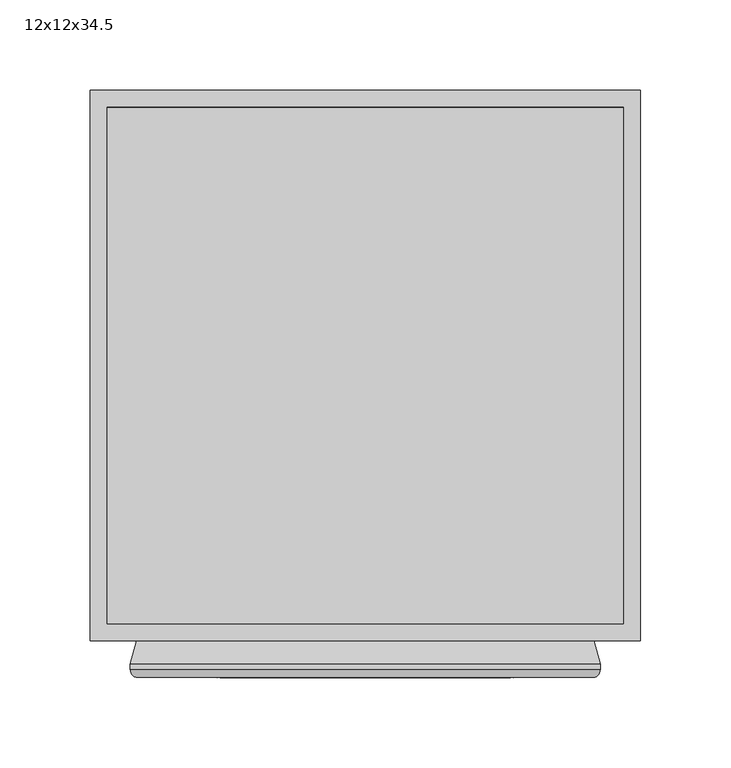
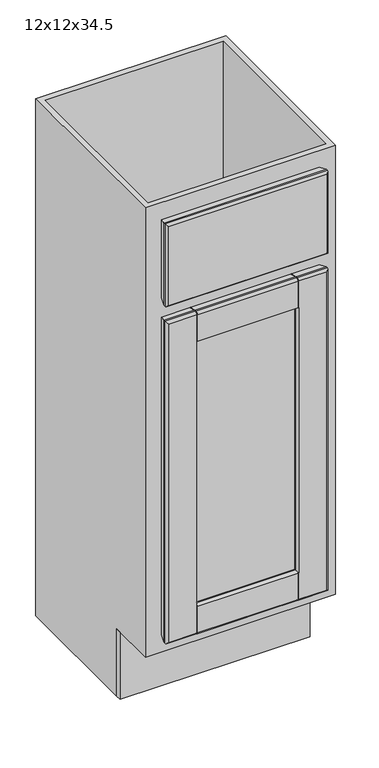
"""IFC4 building model written with IfcOpenShell, lengths in millimetres: furniture geometry, Cabinet-Base-Merillat-Single_Door-Marlin : 12x12x34.5."""

from ifc_helpers import new_model, si_unit, frame, origin, origin_with_axes, place, context, project, spatial, polyline, circle_curve, ellipse_curve, outline, extrude, faceted_brep, source, transform, mapped, element, save
from ifc_brep_helpers import plane_surface, cylinder_surface, advanced_brep


def furniture_12x12x34_5_5e3fd0ca(model_context):
    return source(origin(), model_context, "Body", "SolidModel", [
        advanced_brep(
        [(148.9127049, -625.4496, 685.8), (145.8162124, -629.92, 682.7035075), (145.8162124, -629.92, 142.7964925), (148.9127049, -625.4496, 139.7), (148.9127049, -622.681, 139.7), (148.9127049, -622.681, 685.8), (145.4075049, -609.6, 143.2052), (145.4075049, -609.6, 682.2948), (100.7115422, -609.6, 637.5988372), (100.7115422, -609.6, 187.9011628), (100.3414105, -610.39375, 188.2712945), (98.2602514, -614.85681, 190.3524535), (98.2602514, -614.85681, 635.1475465), (100.3414105, -610.39375, 637.2287055), (99.6600209, -617.0969093, 188.952684), (99.6600209, -617.0969093, 636.547316), (113.9877049, -617.347, 174.625), (113.9877049, -617.347, 650.875), (113.9877049, -622.173, 174.625), (113.9877049, -622.173, 650.875), (99.6600209, -622.4230907, 188.952684), (99.6600209, -622.4230907, 636.547316), (98.2602514, -624.66319, 190.3524535), (98.2602514, -624.66319, 635.1475465), (100.3414105, -629.12625, 188.2712945), (100.7086747, -629.9138508, 187.9040302), (100.7115422, -629.92, 637.5988372), (100.3414105, -629.12625, 637.2287055), (100.7086747, -629.92, 142.7964925), (100.7086747, -625.4496, 139.7), (-108.3408026, -629.92, 142.7964925), (-111.4372951, -625.4496, 139.7), (-63.2730764, -625.4496, 139.7), (-63.2730764, -629.92, 142.7964925), (99.1211747, -625.4496, 139.7), (99.1211747, -629.92, 142.7964925), (-61.6855764, -629.92, 142.7964925), (-61.6855764, -625.4496, 139.7), (100.7086747, -622.681, 139.7), (-111.4372951, -622.681, 139.7), (-63.2730764, -622.681, 139.7), (99.1211747, -622.681, 139.7), (-61.6855764, -622.681, 139.7), (100.7086747, -609.6, 143.2052), (-107.9320951, -609.6, 143.2052), (-63.2730764, -609.6, 143.2052), (99.1211747, -609.6, 143.2052), (-61.6855764, -609.6, 143.2052), (-60.7848416, -614.85681, 190.3524535), (99.1211747, -610.39375, 188.2712945), (99.1211747, -609.6, 187.9011628), (-61.6855764, -609.6, 187.9011628), (-61.6855764, -610.39375, 188.2712945), (-62.8660006, -610.39375, 188.2712945), (-62.184611, -617.0969093, 188.952684), (-76.5122951, -617.347, 174.625), (-76.5122951, -622.173, 174.625), (-62.184611, -622.4230907, 188.952684), (-60.7848416, -624.66319, 190.3524535), (-62.8660006, -629.12625, 188.2712945), (-61.6855764, -629.12625, 188.2712945), (-61.6855764, -629.92, 187.9011628), (99.1211747, -629.92, 187.9011628), (99.1211747, -629.12625, 188.2712945), (-108.3408026, -629.92, 682.7035075), (-111.4372951, -625.4496, 685.8), (-111.4372951, -622.681, 685.8), (-107.9320951, -609.6, 682.2948), (-63.2361323, -609.6, 187.9011628), (-63.2361323, -609.6, 637.5988372), (-62.8660006, -610.39375, 637.2287055), (-60.7848416, -614.85681, 635.1475465), (-62.184611, -617.0969093, 636.547316), (-76.5122951, -617.347, 650.875), (-76.5122951, -622.173, 650.875), (-62.184611, -622.4230907, 636.547316), (-60.7848416, -624.66319, 635.1475465), (-62.8660006, -629.12625, 637.2287055), (-63.2361323, -629.92, 637.5988372), (-63.2361323, -629.92, 187.9011628), (-63.2730764, -629.92, 682.7035075), (-63.2730764, -625.4496, 685.8), (100.7086747, -625.4496, 685.8), (100.7086747, -629.92, 682.7035075), (-61.6855764, -625.4496, 685.8), (-61.6855764, -629.92, 682.7035075), (99.1211747, -629.92, 682.7035075), (99.1211747, -625.4496, 685.8), (-63.2730764, -622.681, 685.8), (100.7086747, -622.681, 685.8), (-61.6855764, -622.681, 685.8), (99.1211747, -622.681, 685.8), (-63.2730764, -609.6, 682.2948), (100.7086747, -609.6, 682.2948), (-61.6855764, -609.6, 682.2948), (99.1211747, -609.6, 682.2948), (-61.6855764, -609.6, 637.5988372), (99.1211747, -609.6, 637.5988372), (-61.6855764, -610.39375, 637.2287055), (99.1211747, -610.39375, 637.2287055), (99.1211747, -629.12625, 637.2287055), (99.1211747, -629.92, 637.5988372), (-61.6855764, -629.92, 637.5988372), (-61.6855764, -629.12625, 637.2287055), (-61.6855764, -610.39375, 681.6857412), (-61.6855764, -622.7855037, 685.00625), (-61.6855764, -625.4496, 685.00625), (-61.6855764, -629.12625, 682.5526052), (-63.2730764, -629.12625, 637.2287055), (-63.2730764, -629.12625, 682.5526052), (-63.2730764, -625.4496, 685.00625), (-63.2730764, -622.7855037, 685.00625), (-63.2730764, -610.39375, 681.6857412), (-63.2730764, -610.39375, 637.2287055), (100.7086747, -610.39375, 637.2287055), (100.7086747, -610.39375, 681.6857412), (100.7086747, -622.7855037, 685.00625), (100.7086747, -625.4496, 685.00625), (100.7086747, -629.12625, 682.5526052), (100.7086747, -629.12625, 637.2287055), (99.1211747, -629.12625, 682.5526052), (99.1211747, -625.4496, 685.00625), (99.1211747, -622.7855037, 685.00625), (99.1211747, -610.39375, 681.6857412), (100.7086747, -629.12625, 188.2712945), (100.7086747, -629.12625, 142.9473948), (100.7086747, -625.4496, 140.49375), (100.7086747, -622.7855037, 140.49375), (100.7086747, -610.39375, 143.8142588), (100.7086747, -610.39375, 188.2712945), (99.1211747, -610.39375, 143.8142588), (99.1211747, -622.7855037, 140.49375), (99.1211747, -625.4496, 140.49375), (99.1211747, -629.12625, 142.9473948), (-61.6855764, -629.12625, 142.9473948), (-61.6855764, -625.4496, 140.49375), (-61.6855764, -622.7855037, 140.49375), (-61.6855764, -610.39375, 143.8142588), (-63.2730764, -629.12625, 188.2712945), (-63.2730764, -610.39375, 188.2712945), (-63.2730764, -610.39375, 143.8142588), (-63.2730764, -622.7855037, 140.49375), (-63.2730764, -625.4496, 140.49375), (-63.2730764, -629.12625, 142.9473948)],
        [
            (0, 1, ellipse_curve(frame((144.1375049, -625.4496, 681.0248), z_axis=(0.7071067811865475, 0.0, -0.7071067811865475), x_axis=(0.7071067811865474, 0.0, 0.7071067811865476)), 6.7531526, 4.7752)),
            (1, 2),
            (2, 3, ellipse_curve(frame((144.1375049, -625.4496, 144.4752), z_axis=(0.7071067811865475, 0.0, 0.7071067811865475), x_axis=(-0.7071067811865474, 0.0, 0.7071067811865476)), 6.7531526, 4.7752)),
            (3, 0),
            (3, 4),
            (4, 5),
            (5, 0),
            (4, 6),
            (6, 7),
            (7, 5),
            (8, 9),
            (9, 10),
            (10, 11),
            (11, 12),
            (12, 13),
            (13, 8),
            (11, 14, ellipse_curve(frame((99.6875049, -615.5223492, 188.9252), z_axis=(0.7071067811865475, 0.0, 0.7071067811865475), x_axis=(-0.7071067811865474, 0.0, 0.7071067811865476)), 2.2271035, 1.5748)),
            (14, 15),
            (15, 12, ellipse_curve(frame((99.6875049, -615.5223492, 636.5748), z_axis=(0.7071067811865475, 0.0, -0.7071067811865475), x_axis=(0.7071067811865474, 0.0, 0.7071067811865476)), 2.2271035, 1.5748)),
            (14, 16),
            (16, 17),
            (17, 15),
            (16, 18),
            (18, 19),
            (19, 17),
            (18, 20),
            (20, 21),
            (21, 19),
            (20, 22, ellipse_curve(frame((99.6875049, -623.9976508, 188.9252), z_axis=(0.7071067811865475, 0.0, 0.7071067811865475), x_axis=(-0.7071067811865474, 0.0, 0.7071067811865476)), 2.2271035, 1.5748)),
            (22, 23),
            (23, 21, ellipse_curve(frame((99.6875049, -623.9976508, 636.5748), z_axis=(0.7071067811865475, 0.0, -0.7071067811865475), x_axis=(0.7071067811865474, 0.0, 0.7071067811865476)), 2.2271035, 1.5748)),
            (22, 24),
            (24, 25),
            (25, 26),
            (26, 27),
            (27, 23),
            (2, 28),
            (28, 29, circle_curve(frame((100.7086747, -625.4496, 144.4752), z_axis=(1.0, 0.0, 0.0), x_axis=(0.0, 1.0, 0.0)), 4.7752)),
            (29, 3),
            (30, 31, ellipse_curve(frame((-106.6620951, -625.4496, 144.4752), z_axis=(0.7071067811865475, 0.0, -0.7071067811865475), x_axis=(0.7071067811865476, 0.0, 0.7071067811865474)), 6.7531526, 4.7752)),
            (31, 32),
            (32, 33, circle_curve(frame((-63.2730764, -625.4496, 144.4752), z_axis=(-1.0, 0.0, 0.0), x_axis=(0.0, 1.0, 0.0)), 4.7752)),
            (33, 30),
            (34, 35, circle_curve(frame((99.1211747, -625.4496, 144.4752), z_axis=(-1.0, 0.0, 0.0), x_axis=(0.0, 1.0, 0.0)), 4.7752)),
            (35, 36),
            (36, 37, circle_curve(frame((-61.6855764, -625.4496, 144.4752), z_axis=(1.0, 0.0, 0.0), x_axis=(0.0, 1.0, 0.0)), 4.7752)),
            (37, 34),
            (29, 38),
            (38, 4),
            (31, 39),
            (39, 40),
            (40, 32),
            (41, 34),
            (37, 42),
            (42, 41),
            (38, 43),
            (43, 6),
            (39, 44),
            (44, 45),
            (45, 40),
            (46, 41),
            (42, 47),
            (47, 46),
            (48, 11),
            (10, 49),
            (49, 50),
            (50, 51),
            (51, 52),
            (52, 53),
            (53, 48),
            (48, 54, ellipse_curve(frame((-62.2120951, -615.5223492, 188.9252), z_axis=(0.7071067811865475, 0.0, -0.7071067811865475), x_axis=(0.7071067811865476, 0.0, 0.7071067811865474)), 2.2271035, 1.5748)),
            (54, 14),
            (54, 55),
            (55, 16),
            (55, 56),
            (56, 18),
            (56, 57),
            (57, 20),
            (57, 58, ellipse_curve(frame((-62.2120951, -623.9976508, 188.9252), z_axis=(0.7071067811865475, 0.0, -0.7071067811865475), x_axis=(0.7071067811865476, 0.0, 0.7071067811865474)), 2.2271035, 1.5748)),
            (58, 22),
            (58, 59),
            (59, 60),
            (60, 61),
            (61, 62),
            (62, 63),
            (63, 24),
            (30, 64),
            (64, 65, ellipse_curve(frame((-106.6620951, -625.4496, 681.0248), z_axis=(-0.7071067811865475, 0.0, -0.7071067811865475), x_axis=(0.7071067811865474, 0.0, -0.7071067811865476)), 6.7531526, 4.7752)),
            (65, 31),
            (65, 66),
            (66, 39),
            (66, 67),
            (67, 44),
            (68, 69),
            (69, 70),
            (70, 71),
            (71, 48),
            (53, 68),
            (71, 72, ellipse_curve(frame((-62.2120951, -615.5223492, 636.5748), z_axis=(-0.7071067811865475, 0.0, -0.7071067811865475), x_axis=(0.7071067811865474, 0.0, -0.7071067811865476)), 2.2271035, 1.5748)),
            (72, 54),
            (72, 73),
            (73, 55),
            (73, 74),
            (74, 56),
            (74, 75),
            (75, 57),
            (75, 76, ellipse_curve(frame((-62.2120951, -623.9976508, 636.5748), z_axis=(-0.7071067811865475, 0.0, -0.7071067811865475), x_axis=(0.7071067811865474, 0.0, -0.7071067811865476)), 2.2271035, 1.5748)),
            (76, 58),
            (76, 77),
            (77, 78),
            (78, 79),
            (79, 59),
            (64, 80),
            (80, 81, circle_curve(frame((-63.2730764, -625.4496, 681.0248), z_axis=(-1.0, 0.0, 0.0), x_axis=(0.0, 1.0, 0.0)), 4.7752)),
            (81, 65),
            (0, 82),
            (82, 83, circle_curve(frame((100.7086747, -625.4496, 681.0248), z_axis=(1.0, 0.0, 0.0), x_axis=(0.0, 1.0, 0.0)), 4.7752)),
            (83, 1),
            (84, 85, circle_curve(frame((-61.6855764, -625.4496, 681.0248), z_axis=(1.0, 0.0, 0.0), x_axis=(0.0, 1.0, 0.0)), 4.7752)),
            (85, 86),
            (86, 87, circle_curve(frame((99.1211747, -625.4496, 681.0248), z_axis=(-1.0, 0.0, 0.0), x_axis=(0.0, 1.0, 0.0)), 4.7752)),
            (87, 84),
            (81, 88),
            (88, 66),
            (5, 89),
            (89, 82),
            (90, 84),
            (87, 91),
            (91, 90),
            (88, 92),
            (92, 67),
            (7, 93),
            (93, 89),
            (94, 90),
            (91, 95),
            (95, 94),
            (43, 9),
            (8, 93),
            (92, 69),
            (68, 45),
            (96, 94),
            (95, 97),
            (97, 96),
            (50, 46),
            (47, 51),
            (12, 71),
            (70, 98),
            (98, 96),
            (97, 99),
            (99, 13),
            (15, 72),
            (17, 73),
            (19, 74),
            (21, 75),
            (23, 76),
            (27, 100),
            (100, 101),
            (101, 102),
            (102, 103),
            (103, 77),
            (83, 26),
            (25, 28),
            (33, 79),
            (78, 80),
            (85, 102),
            (101, 86),
            (35, 62),
            (61, 36),
            (98, 104),
            (104, 105),
            (105, 106),
            (106, 107, circle_curve(frame((-61.6855764, -625.4496, 681.0248), z_axis=(1.0, 0.0, 0.0), x_axis=(0.0, 0.0, 1.0)), 3.98145)),
            (107, 103),
            (78, 108),
            (108, 109),
            (109, 110, circle_curve(frame((-63.2730764, -625.4496, 681.0248), z_axis=(-1.0, 0.0, 0.0), x_axis=(0.0, 0.0, 1.0)), 3.98145)),
            (110, 111),
            (111, 112),
            (112, 113),
            (113, 69),
            (77, 108),
            (107, 109),
            (106, 110),
            (105, 111),
            (104, 112),
            (70, 113),
            (8, 114),
            (114, 115),
            (115, 116),
            (116, 117),
            (117, 118, circle_curve(frame((100.7086747, -625.4496, 681.0248), z_axis=(1.0, 0.0, 0.0), x_axis=(0.0, 0.0, 1.0)), 3.98145)),
            (118, 119),
            (119, 26),
            (100, 120),
            (120, 121, circle_curve(frame((99.1211747, -625.4496, 681.0248), z_axis=(-1.0, 0.0, 0.0), x_axis=(0.0, 0.0, 1.0)), 3.98145)),
            (121, 122),
            (122, 123),
            (123, 99),
            (119, 27),
            (118, 120),
            (117, 121),
            (116, 122),
            (115, 123),
            (114, 13),
            (25, 124),
            (124, 125),
            (125, 126, circle_curve(frame((100.7086747, -625.4496, 144.4752), z_axis=(1.0, 0.0, 0.0), x_axis=(0.0, 0.0, 1.0)), 3.98145)),
            (126, 127),
            (127, 128),
            (128, 129),
            (129, 9),
            (49, 130),
            (130, 131),
            (131, 132),
            (132, 133, circle_curve(frame((99.1211747, -625.4496, 144.4752), z_axis=(-1.0, 0.0, 0.0), x_axis=(0.0, 0.0, 1.0)), 3.98145)),
            (133, 63),
            (129, 10),
            (128, 130),
            (127, 131),
            (126, 132),
            (125, 133),
            (124, 24),
            (60, 134),
            (134, 135, circle_curve(frame((-61.6855764, -625.4496, 144.4752), z_axis=(1.0, 0.0, 0.0), x_axis=(0.0, 0.0, 1.0)), 3.98145)),
            (135, 136),
            (136, 137),
            (137, 52),
            (138, 79),
            (68, 139),
            (139, 140),
            (140, 141),
            (141, 142),
            (142, 143, circle_curve(frame((-63.2730764, -625.4496, 144.4752), z_axis=(-1.0, 0.0, 0.0), x_axis=(0.0, 0.0, 1.0)), 3.98145)),
            (143, 138),
            (138, 59),
            (53, 139),
            (137, 140),
            (136, 141),
            (135, 142),
            (134, 143),
        ],
        [
            cylinder_surface(frame((144.1375049, -625.4496, 685.8), z_axis=(0.0, 0.0, 1.0), x_axis=(0.0, 1.0, 0.0)), 4.7752),
            plane_surface(frame((148.9127049, -625.4496, 685.8), z_axis=(1.0, 0.0, 0.0), x_axis=(0.0, 0.0, -1.0))),
            plane_surface(frame((148.9127049, -622.681, 685.8), z_axis=(0.9659229350723619, 0.25882983502910506, 0.0), x_axis=(0.0, 0.0, -1.0))),
            plane_surface(frame((100.7115422, -609.6, 637.5988372), z_axis=(-0.9063077870366099, 0.4226182617407856, 0.0), x_axis=(0.0, 0.0, -1.0))),
            cylinder_surface(frame((99.6875049, -615.5223492, 685.8), z_axis=(0.0, 0.0, 1.0000000000000002), x_axis=(-0.01745240643729364, -0.9998476951563912, 0.0)), 1.5748),
            plane_surface(frame((99.6600209, -617.0969093, 636.547316), z_axis=(-0.017452406437322144, -0.9998476951563906, 0.0), x_axis=(0.0, 0.0, -1.0))),
            plane_surface(frame((113.9877049, -617.347, 650.875), z_axis=(-1.0, 0.0, 0.0), x_axis=(0.0, 0.0, -1.0))),
            plane_surface(frame((113.9877049, -622.173, 650.875), z_axis=(-0.01745240643727848, 0.9998476951563914, 0.0), x_axis=(0.0, 0.0, -1.0))),
            cylinder_surface(frame((99.6875049, -623.9976508, 685.8), z_axis=(0.0, 0.0, 1.0000000000000002), x_axis=(-0.9063077870367326, -0.42261826174052236, 0.0)), 1.5748),
            plane_surface(frame((98.2602514, -624.66319, 635.1475465), z_axis=(-0.9063077870366333, -0.4226182617407352, 0.0), x_axis=(0.0, 0.0, -1.0))),
            cylinder_surface(frame((148.9127049, -625.4496, 144.4752), z_axis=(1.0, 0.0, 0.0), x_axis=(0.0, 1.0, 0.0)), 4.7752),
            plane_surface(frame((148.9127049, -625.4496, 139.7), z_axis=(0.0, 0.0, -1.0), x_axis=(-1.0, 0.0, 0.0))),
            plane_surface(frame((148.9127049, -622.681, 139.7), z_axis=(0.0, 0.25882983502910506, -0.9659229350723619), x_axis=(-1.0, 0.0, 0.0))),
            plane_surface(frame((100.7115422, -609.6, 187.9011628), z_axis=(0.0, 0.4226182617407856, 0.9063077870366099), x_axis=(-1.0, 0.0, 0.0))),
            cylinder_surface(frame((148.9127049, -615.5223492, 188.9252), z_axis=(1.0000000000000002, 0.0, 0.0), x_axis=(0.0, -0.9998476951563912, 0.01745240643729364)), 1.5748),
            plane_surface(frame((99.6600209, -617.0969093, 188.952684), z_axis=(0.0, -0.9998476951563906, 0.017452406437322144), x_axis=(-1.0, 0.0, 0.0))),
            plane_surface(frame((113.9877049, -617.347, 174.625), z_axis=(0.0, 0.0, 1.0), x_axis=(-1.0, 0.0, 0.0))),
            plane_surface(frame((113.9877049, -622.173, 174.625), z_axis=(0.0, 0.9998476951563914, 0.01745240643727848), x_axis=(-1.0, 0.0, 0.0))),
            cylinder_surface(frame((148.9127049, -623.9976508, 188.9252), z_axis=(1.0000000000000002, 0.0, 0.0), x_axis=(0.0, -0.42261826174052236, 0.9063077870367326)), 1.5748),
            plane_surface(frame((98.2602514, -624.66319, 190.3524535), z_axis=(0.0, -0.4226182617407352, 0.9063077870366333), x_axis=(-1.0, 0.0, 0.0))),
            cylinder_surface(frame((-106.6620951, -625.4496, 139.7), z_axis=(0.0, 0.0, -1.0), x_axis=(0.0, 1.0, 0.0)), 4.7752),
            plane_surface(frame((-111.4372951, -625.4496, 139.7), z_axis=(-1.0, 0.0, 0.0), x_axis=(0.0, 0.0, 1.0))),
            plane_surface(frame((-111.4372951, -622.681, 139.7), z_axis=(-0.9659229350723619, 0.25882983502910506, 0.0), x_axis=(0.0, 0.0, 1.0))),
            plane_surface(frame((-63.2361323, -609.6, 187.9011628), z_axis=(0.9063077870366099, 0.4226182617407856, 0.0), x_axis=(0.0, 0.0, 1.0))),
            cylinder_surface(frame((-62.2120951, -615.5223492, 139.7), z_axis=(0.0, 0.0, -1.0000000000000002), x_axis=(0.01745240643729364, -0.9998476951563912, 0.0)), 1.5748),
            plane_surface(frame((-62.184611, -617.0969093, 188.952684), z_axis=(0.017452406437322144, -0.9998476951563906, 0.0), x_axis=(0.0, 0.0, 1.0))),
            plane_surface(frame((-76.5122951, -617.347, 174.625), z_axis=(1.0, 0.0, 0.0), x_axis=(0.0, 0.0, 1.0))),
            plane_surface(frame((-76.5122951, -622.173, 174.625), z_axis=(0.01745240643727848, 0.9998476951563914, 0.0), x_axis=(0.0, 0.0, 1.0))),
            cylinder_surface(frame((-62.2120951, -623.9976508, 139.7), z_axis=(0.0, 0.0, -1.0000000000000002), x_axis=(0.9063077870367326, -0.42261826174052236, 0.0)), 1.5748),
            plane_surface(frame((-60.7848416, -624.66319, 190.3524535), z_axis=(0.9063077870366333, -0.4226182617407352, 0.0), x_axis=(0.0, 0.0, 1.0))),
            cylinder_surface(frame((-111.4372951, -625.4496, 681.0248), z_axis=(-1.0, 0.0, 0.0), x_axis=(0.0, 1.0, 0.0)), 4.7752),
            plane_surface(frame((-111.4372951, -625.4496, 685.8), z_axis=(0.0, 0.0, 1.0), x_axis=(1.0, 0.0, 0.0))),
            plane_surface(frame((-111.4372951, -622.681, 685.8), z_axis=(0.0, 0.25882983502910506, 0.9659229350723619), x_axis=(1.0, 0.0, 0.0))),
            plane_surface(frame((-107.9320951, -609.6, 682.2948), z_axis=(0.0, 1.0, 0.0), x_axis=(1.0, 0.0, 0.0))),
            plane_surface(frame((-63.2361323, -609.6, 637.5988372), z_axis=(0.0, 0.4226182617407856, -0.9063077870366099), x_axis=(1.0, 0.0, 0.0))),
            cylinder_surface(frame((-111.4372951, -615.5223492, 636.5748), z_axis=(-1.0000000000000002, 0.0, 0.0), x_axis=(0.0, -0.9998476951563912, -0.01745240643729364)), 1.5748),
            plane_surface(frame((-62.184611, -617.0969093, 636.547316), z_axis=(0.0, -0.9998476951563906, -0.017452406437322144), x_axis=(1.0, 0.0, 0.0))),
            plane_surface(frame((-76.5122951, -617.347, 650.875), z_axis=(0.0, 0.0, -1.0), x_axis=(1.0, 0.0, 0.0))),
            plane_surface(frame((-76.5122951, -622.173, 650.875), z_axis=(0.0, 0.9998476951563914, -0.01745240643727848), x_axis=(1.0, 0.0, 0.0))),
            cylinder_surface(frame((-111.4372951, -623.9976508, 636.5748), z_axis=(-1.0000000000000002, 0.0, 0.0), x_axis=(0.0, -0.42261826174052236, -0.9063077870367326)), 1.5748),
            plane_surface(frame((-60.7848416, -624.66319, 635.1475465), z_axis=(0.0, -0.4226182617407352, -0.9063077870366333), x_axis=(1.0, 0.0, 0.0))),
            plane_surface(frame((-63.2361323, -629.92, 637.5988372), z_axis=(0.0, -1.0, 0.0), x_axis=(1.0, 0.0, 0.0))),
            plane_surface(frame((-61.6855764, -629.92, 637.5988372), z_axis=(-1.0, 0.0, 0.0), x_axis=(0.0, 0.906307787036771, -0.4226182617404399))),
            plane_surface(frame((-63.2730764, -629.92, 637.5988372), z_axis=(1.0, 0.0, 0.0), x_axis=(0.0, -0.906307787036771, 0.4226182617404399))),
            plane_surface(frame((-61.6855764, -629.92, 637.5988372), z_axis=(0.0, 0.4226182617404399, 0.906307787036771), x_axis=(-1.0, 0.0, 0.0))),
            plane_surface(frame((-61.6855764, -629.12625, 637.2287055), z_axis=(0.0, -1.0, 0.0), x_axis=(-1.0, 0.0, 0.0))),
            cylinder_surface(frame((-63.2730764, -625.4496, 681.0248), z_axis=(-1.0, 0.0, 0.0), x_axis=(0.0, 0.0, 1.0)), 3.98145),
            plane_surface(frame((-61.6855764, -625.4496, 685.00625), z_axis=(0.0, 0.0, 1.0), x_axis=(-1.0, 0.0, 0.0))),
            plane_surface(frame((-61.6855764, -622.7855037, 685.00625), z_axis=(0.0, 0.25882983502913415, 0.9659229350723542), x_axis=(-1.0, 0.0, 0.0))),
            plane_surface(frame((-61.6855764, -610.39375, 681.6857412), z_axis=(0.0, 1.0, 0.0), x_axis=(-1.0, 0.0, 0.0))),
            plane_surface(frame((-61.6855764, -610.39375, 637.2287055), z_axis=(0.0, -0.4226182617405111, 0.9063077870367379), x_axis=(-1.0, 0.0, 0.0))),
            plane_surface(frame((100.7086747, -629.92, 637.5988372), z_axis=(-1.0, 0.0, 0.0), x_axis=(0.0, 0.9063077870367783, -0.42261826174042444))),
            plane_surface(frame((99.1211747, -629.92, 637.5988372), z_axis=(1.0, 0.0, 0.0), x_axis=(0.0, -0.9063077870367783, 0.42261826174042444))),
            plane_surface(frame((100.7086747, -629.92, 637.5988372), z_axis=(0.0, 0.42261826174042444, 0.9063077870367783), x_axis=(-1.0, 0.0, 0.0))),
            plane_surface(frame((100.7086747, -629.12625, 637.2287055), z_axis=(0.0, -1.0, 0.0), x_axis=(-1.0, 0.0, 0.0))),
            cylinder_surface(frame((99.1211747, -625.4496, 681.0248), z_axis=(-1.0, 0.0, 0.0), x_axis=(0.0, 0.0, 1.0)), 3.98145),
            plane_surface(frame((100.7086747, -625.4496, 685.00625), z_axis=(0.0, 0.0, 1.0), x_axis=(-1.0, 0.0, 0.0))),
            plane_surface(frame((100.7086747, -622.7855037, 685.00625), z_axis=(0.0, 0.25882983502911566, 0.965922935072359), x_axis=(-1.0, 0.0, 0.0))),
            plane_surface(frame((100.7086747, -610.39375, 681.6857412), z_axis=(0.0, 1.0, 0.0), x_axis=(-1.0, 0.0, 0.0))),
            plane_surface(frame((100.7086747, -610.39375, 637.2287055), z_axis=(0.0, -0.42261826174056427, 0.9063077870367131), x_axis=(-1.0, 0.0, 0.0))),
            plane_surface(frame((100.7086747, -625.4496, 149.2504), z_axis=(-1.0, 0.0, 0.0), x_axis=(0.0, -1.0, 0.0))),
            plane_surface(frame((99.1211747, -625.4496, 149.2504), z_axis=(1.0, 0.0, 0.0), x_axis=(0.0, 1.0, 0.0))),
            plane_surface(frame((100.7086747, -609.6, 187.9011628), z_axis=(0.0, -0.42261826173999295, -0.9063077870369795), x_axis=(-1.0, 0.0, 0.0))),
            plane_surface(frame((100.7086747, -610.39375, 188.2712945), z_axis=(0.0, 1.0, 0.0), x_axis=(-1.0, 0.0, 0.0))),
            plane_surface(frame((100.7086747, -610.39375, 143.8142588), z_axis=(0.0, 0.2588298350290845, -0.9659229350723675), x_axis=(-1.0, 0.0, 0.0))),
            plane_surface(frame((100.7086747, -622.7855037, 140.49375), z_axis=(0.0, 0.0, -1.0), x_axis=(-1.0, 0.0, 0.0))),
            cylinder_surface(frame((99.1211747, -625.4496, 144.4752), z_axis=(-1.0, 0.0, 0.0), x_axis=(0.0, 0.0, 1.0)), 3.98145),
            plane_surface(frame((100.7086747, -629.12625, 142.9473948), z_axis=(0.0, -1.0, 0.0), x_axis=(-1.0, 0.0, 0.0))),
            plane_surface(frame((100.7086747, -629.12625, 188.2712945), z_axis=(0.0, 0.4226182617407698, -0.9063077870366172), x_axis=(-1.0, 0.0, 0.0))),
            plane_surface(frame((-61.6855764, -629.12625, 188.2712945), z_axis=(-1.0, 0.0, 0.0), x_axis=(0.0, -0.906307787036583, -0.42261826174084305))),
            plane_surface(frame((-63.2730764, -629.12625, 188.2712945), z_axis=(1.0, 0.0, 0.0), x_axis=(0.0, 0.906307787036583, 0.42261826174084305))),
            plane_surface(frame((-61.6855764, -629.12625, 188.2712945), z_axis=(0.0, 0.42261826174084305, -0.906307787036583), x_axis=(-1.0, 0.0, 0.0))),
            plane_surface(frame((-61.6855764, -609.6, 187.9011628), z_axis=(0.0, -0.42261826174073325, -0.9063077870366342), x_axis=(-1.0, 0.0, 0.0))),
            plane_surface(frame((-61.6855764, -610.39375, 188.2712945), z_axis=(0.0, 1.0, 0.0), x_axis=(-1.0, 0.0, 0.0))),
            plane_surface(frame((-61.6855764, -610.39375, 143.8142588), z_axis=(0.0, 0.2588298350290967, -0.9659229350723642), x_axis=(-1.0, 0.0, 0.0))),
            plane_surface(frame((-61.6855764, -622.7855037, 140.49375), z_axis=(0.0, 0.0, -1.0), x_axis=(-1.0, 0.0, 0.0))),
            cylinder_surface(frame((-63.2730764, -625.4496, 144.4752), z_axis=(-1.0, 0.0, 0.0), x_axis=(0.0, 0.0, 1.0)), 3.98145),
            plane_surface(frame((-61.6855764, -629.12625, 142.9473948), z_axis=(0.0, -1.0, 0.0), x_axis=(-1.0, 0.0, 0.0))),
        ],
        [
            (0, [[1, 2, 3, 4]]),
            (1, [[-4, 5, 6, 7]]),
            (2, [[-6, 8, 9, 10]]),
            (3, [[11, 12, 13, 14, 15, 16]]),
            (4, [[-14, 17, 18, 19]]),
            (5, [[-18, 20, 21, 22]]),
            (6, [[-21, 23, 24, 25]]),
            (7, [[-24, 26, 27, 28]]),
            (8, [[-27, 29, 30, 31]]),
            (9, [[-30, 32, 33, 34, 35, 36]]),
            (10, [[-3, 37, 38, 39]]),
            (10, [[40, 41, 42, 43]]),
            (10, [[44, 45, 46, 47]]),
            (11, [[-5, -39, 48, 49]]),
            (11, [[50, 51, 52, -41]]),
            (11, [[53, -47, 54, 55]]),
            (12, [[-8, -49, 56, 57]]),
            (12, [[58, 59, 60, -51]]),
            (12, [[61, -55, 62, 63]]),
            (13, [[64, -13, 65, 66, 67, 68, 69, 70]]),
            (14, [[-17, -64, 71, 72]]),
            (15, [[-20, -72, 73, 74]]),
            (16, [[-23, -74, 75, 76]]),
            (17, [[-26, -76, 77, 78]]),
            (18, [[-29, -78, 79, 80]]),
            (19, [[-80, 81, 82, 83, 84, 85, 86, -32]]),
            (20, [[-40, 87, 88, 89]]),
            (21, [[-50, -89, 90, 91]]),
            (22, [[-58, -91, 92, 93]]),
            (23, [[94, 95, 96, 97, -70, 98]]),
            (24, [[-71, -97, 99, 100]]),
            (25, [[-73, -100, 101, 102]]),
            (26, [[-75, -102, 103, 104]]),
            (27, [[-77, -104, 105, 106]]),
            (28, [[-79, -106, 107, 108]]),
            (29, [[-108, 109, 110, 111, 112, -81]]),
            (30, [[-88, 113, 114, 115]]),
            (30, [[-1, 116, 117, 118]]),
            (30, [[119, 120, 121, 122]]),
            (31, [[-90, -115, 123, 124]]),
            (31, [[-7, 125, 126, -116]]),
            (31, [[127, -122, 128, 129]]),
            (32, [[-92, -124, 130, 131]]),
            (32, [[-10, 132, 133, -125]]),
            (32, [[134, -129, 135, 136]]),
            (33, [[-9, -57, 137, -11, 138, -132]]),
            (33, [[-93, -131, 139, -94, 140, -59]]),
            (33, [[141, -136, 142, 143]]),
            (33, [[144, -63, 145, -67]]),
            (34, [[146, -96, 147, 148, -143, 149, 150, -15]]),
            (35, [[-19, 151, -99, -146]]),
            (36, [[-22, 152, -101, -151]]),
            (37, [[-25, 153, -103, -152]]),
            (38, [[-28, 154, -105, -153]]),
            (39, [[-31, 155, -107, -154]]),
            (40, [[-155, -36, 156, 157, 158, 159, 160, -109]]),
            (41, [[-2, -118, 161, -34, 162, -37]]),
            (41, [[-87, -43, 163, -111, 164, -113]]),
            (41, [[165, -158, 166, -120]]),
            (41, [[167, -84, 168, -45]]),
            (42, [[169, 170, 171, 172, 173, -159, -165, -119, -127, -134, -141, -148]]),
            (43, [[174, 175, 176, 177, 178, 179, 180, -139, -130, -123, -114, -164]]),
            (44, [[-174, -110, 181]]),
            (45, [[-173, 182, -175, -181, -160]]),
            (46, [[-172, 183, -176, -182]]),
            (47, [[-171, 184, -177, -183]]),
            (48, [[-170, 185, -178, -184]]),
            (49, [[-169, -147, 186, -179, -185]]),
            (50, [[-180, -186, -95]]),
            (51, [[187, 188, 189, 190, 191, 192, 193, -161, -117, -126, -133, -138]]),
            (52, [[194, 195, 196, 197, 198, -149, -142, -135, -128, -121, -166, -157]]),
            (53, [[-193, 199, -35]]),
            (54, [[-192, 200, -194, -156, -199]]),
            (55, [[-191, 201, -195, -200]]),
            (56, [[-190, 202, -196, -201]]),
            (57, [[-189, 203, -197, -202]]),
            (58, [[-188, 204, -150, -198, -203]]),
            (59, [[-187, -16, -204]]),
            (60, [[205, 206, 207, 208, 209, 210, 211, -137, -56, -48, -38, -162]]),
            (61, [[212, 213, 214, 215, 216, -85, -167, -44, -53, -61, -144, -66]]),
            (62, [[-211, 217, -12]]),
            (63, [[-210, 218, -212, -65, -217]]),
            (64, [[-209, 219, -213, -218]]),
            (65, [[-208, 220, -214, -219]]),
            (66, [[-207, 221, -215, -220]]),
            (67, [[-206, 222, -86, -216, -221]]),
            (68, [[-205, -33, -222]]),
            (69, [[223, 224, 225, 226, 227, -68, -145, -62, -54, -46, -168, -83]]),
            (70, [[228, -163, -42, -52, -60, -140, 229, 230, 231, 232, 233, 234]]),
            (71, [[-228, 235, -112]]),
            (72, [[-229, -98, 236]]),
            (73, [[-227, 237, -230, -236, -69]]),
            (74, [[-226, 238, -231, -237]]),
            (75, [[-225, 239, -232, -238]]),
            (76, [[-224, 240, -233, -239]]),
            (77, [[-223, -82, -235, -234, -240]]),
        ],
    ),
        extrude(outline(polyline([(-76.5122951, -622.173), (-76.5122951, -617.347), (113.9877049, -617.347), (113.9877049, -622.173), (-76.5122951, -622.173)])), frame((0.0, 0.0, 174.625), z_axis=(0.0, 0.0, 1.0), x_axis=(1.0, 0.0, 0.0)), (0.0, 0.0, 1.0), 476.25),
        advanced_brep(
        [(-108.3408026, -629.92, 847.8035075), (-108.3408026, -629.92, 714.2964925), (145.8162124, -629.92, 714.2964925), (145.8162124, -629.92, 847.8035075), (-107.9320951, -609.6, 714.7052), (-107.9320951, -609.6, 847.3948), (145.4075049, -609.6, 847.3948), (145.4075049, -609.6, 714.7052), (-111.4372951, -625.4496, 850.9), (-111.4372951, -622.681, 850.9), (-111.4372951, -622.681, 711.2), (-111.4372951, -625.4496, 711.2), (148.9127049, -622.681, 711.2), (148.9127049, -625.4496, 711.2), (148.9127049, -622.681, 850.9), (148.9127049, -625.4496, 850.9)],
        [
            (0, 1),
            (1, 2),
            (2, 3),
            (3, 0),
            (4, 5),
            (5, 6),
            (6, 7),
            (7, 4),
            (8, 9),
            (9, 10),
            (10, 11),
            (11, 8),
            (10, 12),
            (12, 13),
            (13, 11),
            (12, 14),
            (14, 15),
            (15, 13),
            (8, 15),
            (14, 9),
            (11, 1, ellipse_curve(frame((-106.6620951, -625.4496, 715.9752), z_axis=(-0.7071067811865475, 0.0, 0.7071067811865475), x_axis=(-0.7071067811865474, 0.0, -0.7071067811865476)), 6.7531526, 4.7752)),
            (0, 8, ellipse_curve(frame((-106.6620951, -625.4496, 846.1248), z_axis=(-0.7071067811865475, 0.0, -0.7071067811865475), x_axis=(0.7071067811865474, 0.0, -0.7071067811865476)), 6.7531526, 4.7752)),
            (4, 10),
            (9, 5),
            (13, 2, ellipse_curve(frame((144.1375049, -625.4496, 715.9752), z_axis=(-0.7071067811865475, 0.0, -0.7071067811865475), x_axis=(0.7071067811865476, 0.0, -0.7071067811865474)), 6.7531526, 4.7752)),
            (7, 12),
            (15, 3, ellipse_curve(frame((144.1375049, -625.4496, 846.1248), z_axis=(0.7071067811865475, 0.0, -0.7071067811865475), x_axis=(0.7071067811865474, 0.0, 0.7071067811865476)), 6.7531526, 4.7752)),
            (6, 14),
        ],
        [
            plane_surface(frame((-111.4372951, -629.92, 850.9), z_axis=(0.0, -1.0, 0.0), x_axis=(0.0, 0.0, -1.0))),
            plane_surface(frame((-111.4372951, -609.6, 850.9), z_axis=(0.0, 1.0, 0.0), x_axis=(0.0, 0.0, 1.0))),
            plane_surface(frame((-111.4372951, -629.92, 850.9), z_axis=(-1.0, 0.0, 0.0), x_axis=(0.0, 1.0, 0.0))),
            plane_surface(frame((-111.4372951, -629.92, 711.2), z_axis=(0.0, 0.0, -1.0), x_axis=(0.0, 1.0, 0.0))),
            plane_surface(frame((148.9127049, -629.92, 711.2), z_axis=(1.0, 0.0, 0.0), x_axis=(0.0, 1.0, 0.0))),
            plane_surface(frame((148.9127049, -629.92, 850.9), z_axis=(0.0, 0.0, 1.0), x_axis=(0.0, 1.0, 0.0))),
            cylinder_surface(frame((-106.6620951, -625.4496, 850.9), z_axis=(0.0, 0.0, -1.0), x_axis=(0.0, 1.0, 0.0)), 4.7752),
            plane_surface(frame((-111.4372951, -622.681, 850.9), z_axis=(-0.9659229350723619, 0.25882983502910506, 0.0), x_axis=(0.0, 0.0, -1.0))),
            cylinder_surface(frame((-111.4372951, -625.4496, 715.9752), z_axis=(1.0, 0.0, 0.0), x_axis=(0.0, 1.0, 0.0)), 4.7752),
            plane_surface(frame((-111.4372951, -622.681, 711.2), z_axis=(0.0, 0.25882983502910506, -0.9659229350723619), x_axis=(1.0, 0.0, 0.0))),
            cylinder_surface(frame((144.1375049, -625.4496, 711.2), z_axis=(0.0, 0.0, 1.0), x_axis=(0.0, 1.0, 0.0)), 4.7752),
            plane_surface(frame((148.9127049, -622.681, 711.2), z_axis=(0.9659229350723619, 0.25882983502910506, 0.0), x_axis=(0.0, 0.0, 1.0))),
            cylinder_surface(frame((148.9127049, -625.4496, 846.1248), z_axis=(-1.0, 0.0, 0.0), x_axis=(0.0, 1.0, 0.0)), 4.7752),
            plane_surface(frame((148.9127049, -622.681, 850.9), z_axis=(0.0, 0.25882983502910506, 0.9659229350723619), x_axis=(-1.0, 0.0, 0.0))),
        ],
        [
            (0, [[1, 2, 3, 4]]),
            (1, [[5, 6, 7, 8]]),
            (2, [[9, 10, 11, 12]]),
            (3, [[-11, 13, 14, 15]]),
            (4, [[-14, 16, 17, 18]]),
            (5, [[-9, 19, -17, 20]]),
            (6, [[21, -1, 22, -12]]),
            (7, [[23, -10, 24, -5]]),
            (8, [[-21, -15, 25, -2]]),
            (9, [[-23, -8, 26, -13]]),
            (10, [[-25, -18, 27, -3]]),
            (11, [[-26, -7, 28, -16]]),
            (12, [[-22, -4, -27, -19]]),
            (13, [[-24, -20, -28, -6]]),
        ],
    ),
        extrude(outline(polyline([(-133.6622951, -538.95625), (-133.6622951, -529.43125), (171.1377049, -529.43125), (171.1377049, -538.95625), (-133.6622951, -538.95625)])), origin_with_axes(), (0.0, 0.0, 1.0), 114.3),
        faceted_brep([(171.1377049, -304.8, 0.0), (171.1377049, -529.43125, 0.0), (161.6127049, -529.43125, 0.0), (161.6127049, -314.325, 0.0), (-124.1372951, -314.325, 0.0), (-124.1372951, -529.43125, 0.0), (-133.6622951, -529.43125, 0.0), (-133.6622951, -304.8, 0.0), (-133.6622951, -304.8, 876.3), (171.1377049, -304.8, 876.3), (-133.6622951, -529.43125, 114.3), (-133.6622951, -609.6, 114.3), (-133.6622951, -609.6, 876.3), (171.1377049, -609.6, 876.3), (171.1377049, -609.6, 114.3), (171.1377049, -529.43125, 114.3), (161.6127049, -529.43125, 114.3), (161.6127049, -314.325, 114.3), (161.6127049, -600.075, 876.3), (161.6127049, -314.325, 876.3), (161.6127049, -314.325, 119.0625), (161.6127049, -600.075, 119.0625), (-124.1372951, -529.43125, 114.3), (-124.1372951, -314.325, 114.3), (-124.1372951, -314.325, 876.3), (-124.1372951, -600.075, 876.3), (-124.1372951, -600.075, 119.0625), (-124.1372951, -314.325, 119.0625)], [[[0, 1, 2, 3, 4, 5, 6, 7]], [[0, 7, 8, 9]], [[7, 6, 10, 11, 12, 8]], [[1, 0, 9, 13, 14, 15]], [[3, 2, 16, 17]], [[18, 19, 20, 21]], [[6, 5, 22, 10]], [[5, 4, 23, 22]], [[24, 25, 26, 27]], [[4, 3, 17, 23]], [[19, 24, 27, 20]], [[9, 8, 12, 13], [19, 18, 25, 24]], [[14, 11, 10, 22, 23, 17, 16, 15]], [[13, 12, 11, 14]], [[25, 18, 21, 26]], [[21, 20, 27, 26]], [[2, 1, 15, 16]]]),
    ])


if __name__ == "__main__":
    model = new_model("IFC4")
    model_context = context("Model", 3, world=origin())
    ifc_project = project(units=[si_unit("LENGTHUNIT", "METRE", prefix="MILLI")], contexts=[model_context])
    site = spatial("IfcSite", under=ifc_project)
    building = spatial("IfcBuilding", under=site)
    placement = place(None, origin())
    furniture_12x12x34_5_shape = furniture_12x12x34_5_5e3fd0ca(model_context)
    element("IfcFurniture", 1, ObjectType="Cabinet-Base-Merillat-Single_Door-Marlin : 12x12x34.5", at=placement, inside=building, context=model_context, shape_type="MappedRepresentation", body=[
        mapped(furniture_12x12x34_5_shape, transform((0.0, 0.0, 0.0), x_axis=(1.0, 0.0, 0.0), y_axis=(0.0, 1.0, 0.0), z_axis=(0.0, 0.0, 1.0))),
    ])
    save(model, "model.ifc")

# Revit data of these elements
# Type "Cabinet-Base-Merillat-Single_Door-Marlin : 12x12x34.5"
#   URL = "http://www.merillat.com"
#   Toe Kick Note = "Toe Kick Covering is not included. To be purchased Separately."
#   Product Page URL = "http://www.merillat.com//our-products/rooms/kitchen/"
#   Product Line = "Express"
#   Product Group = "Base Cabinet"
#   Product Documentation Link = "http://merillatbusiness.com/customer-resources/product-line-resources/merillat-classic/"
#   Model = "SB12 R or L"
#   Manufacturer = "Merillat"
#   Finish = "Wood"
#   Description = "Sink Base Single Door/Drawer"
#   Construction Type = "Sink Base Single Door"
#   Cabinet Construction Note = "No shelf, One full-width false drawer front, Specify R or L"
#   Assembly Code = "C1030410"
#   Top and Bottom Spacing = 0' - 1"
#   Toe Kick Height = 0' - 4 1/2"
#   Toe Kick Depth = 0' - 2 25/32"
#   Depth = 1' - 0"
#   Height = 2' - 10 1/2"
#   Width = 1' - 0"
#   Cabinet Shell = 0' - 0 3/8"
#   Cabinet Drawer Width = 0' - 10 1/4"
#   Cabinet Drawer Height = 0' - 5 1/2"
#   Cabinet Door Width = 0' - 10 1/4"
#   Cabinet Door Height = 1' - 9 1/2"
#   COBie.Type = no
#   Partial Overlay = yes
#   Full Overlay = no
#   Elevation Swing Line = yes
#   Toe Kick Material = Wood - Merillat - Raw Particle Board
#   Door Drawer Material = Wood - Merillat - Pecan(1)
#   Cabinet Material = Wood - Merillat - Pecan(1)
#   Cabinet Drawer Style = element 785883
#   Cabinet Door Style = element 785884
# Element 1 (IfcFurniture, "Cabinet-Base-Merillat-Single_Door-Marlin : 12x12x34.5")
#   Materials on its faces: "Wood - Merillat - Pecan(1)", "Wood - Merillat - Raw Particle Board"
# Materials
#   "Wood - Merillat - Raw Particle Board": class "Plastic", colour RGB 80 80 80, transparency 0, Description = "Plastic Laminate - Navy", Cost = 0
#   "Wood - Merillat - Pecan(1)": class "Wood", colour RGB 108 67 43, transparency 0, Cost = 0
